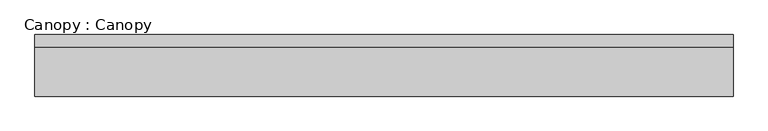
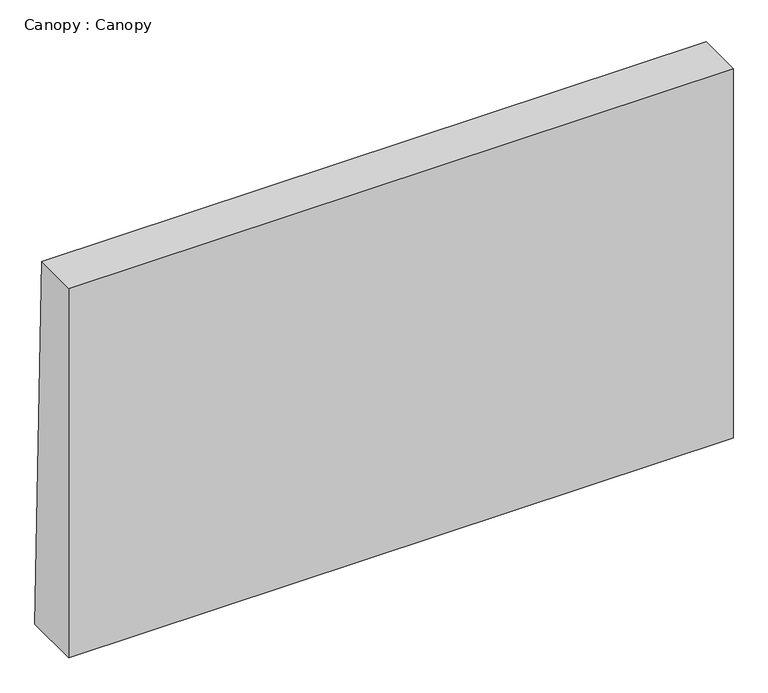
"""IFC4 building model written with IfcOpenShell, lengths in millimetres: proxy geometry, Canopy : Canopy."""

from ifc_helpers import new_model, si_unit, frame, origin, place, context, project, spatial, polyline, outline, extrude, source, transform, mapped, element, save


def canopy_canopy_239b8731(model_context):
    return source(origin(), model_context, "Body", "SweptSolid", [
        extrude(outline(polyline([(150.0, 0.0), (0.0, 0.0), (0.0, 1000.0), (120.0, 1000.0), (150.0, 0.0)])), frame((-850.0, 0.0, 0.0), z_axis=(1.0, 0.0, 0.0), x_axis=(0.0, 1.0, 0.0)), (0.0, 0.0, 1.0), 1700.0),
    ])


if __name__ == "__main__":
    model = new_model("IFC4")
    model_context = context("Model", 3, world=origin())
    ifc_project = project(units=[si_unit("LENGTHUNIT", "METRE", prefix="MILLI")], contexts=[model_context])
    site = spatial("IfcSite", under=ifc_project)
    building = spatial("IfcBuilding", under=site)
    placement = place(None, origin())
    canopy_canopy_shape = canopy_canopy_239b8731(model_context)
    element("IfcBuildingElementProxy", 1, Name="Canopy : Canopy", ObjectType="Canopy : Canopy", at=placement, inside=building, context=model_context, shape_type="MappedRepresentation", body=[
        mapped(canopy_canopy_shape, transform((0.0, 0.0, 0.0), x_axis=(1.0, 0.0, 0.0), y_axis=(0.0, 1.0, 0.0), z_axis=(0.0, 0.0, 1.0))),
    ])
    save(model, "model.ifc")

# Revit data of these elements
# Type "Canopy : Canopy"
#   Type Comments = "CV-AG"
#   H_Rebar Ratio = 0.1
#   Canopy Width [instance default] = 1700 mm
#   Canopy Length [instance default] = 1000 mm
#   Canopy L.P = 120 mm
#   Canopy H.P = 150 mm
#   구조재료 = Concrete_f'c=28MPa(Cylender)
#   Default Elevation = 0
# Element 1 (IfcBuildingElementProxy, "Canopy : Canopy")
#   Materials on its faces: "Concrete_f'c=28MPa(Cylender)"
# Materials
#   "Concrete_f'c=28MPa(Cylender)": class "Concrete", colour RGB 176 176 176, transparency 0, Description = "Reinf. Conc.", Cost = 0, Image = Concrete.Cast-In-Place.Flat.Polished.Grey.jpg
